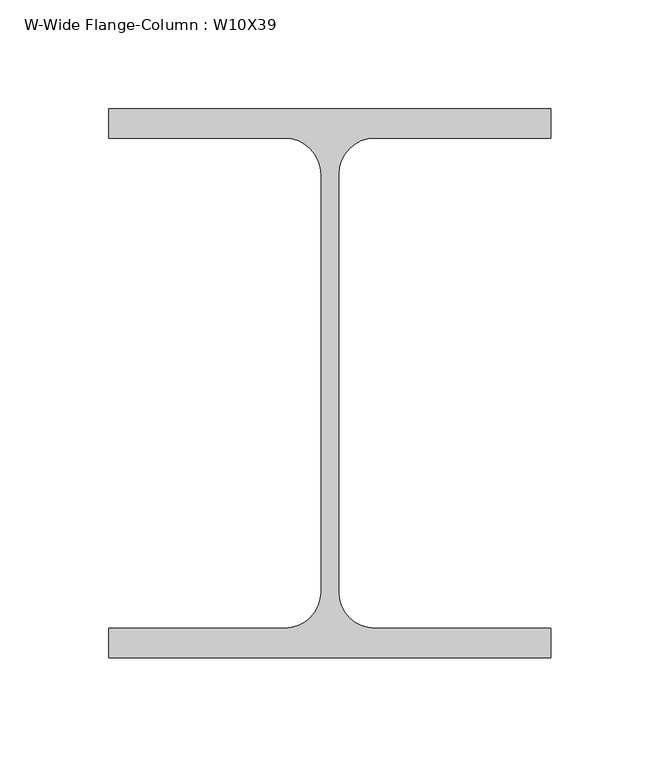
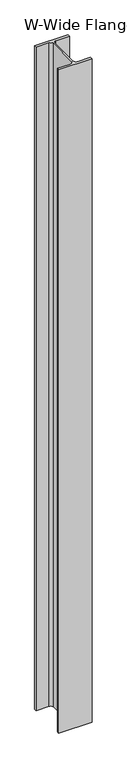
"""IFC4 building model written with IfcOpenShell, lengths in millimetres: column geometry, W-Wide Flange-Column : W10X39."""

from ifc_helpers import new_model, si_unit, point, frame, frame_2d, origin, place, context, project, spatial, polyline, circle_curve, trimmed, segment, composite_curve, outline, extrude, source, transform, mapped, element, save


def w_wide_flange_column_w10x39_5a593fdc(model_context):
    return source(origin(), model_context, "Body", "SweptSolid", [
        extrude(outline(composite_curve([segment(polyline([(101.473, 125.984), (101.473, 112.522), (20.701, 112.522)]), True, "CONTINUOUS"), segment(trimmed(circle_curve(frame_2d((20.701, 95.8215)), 16.7005), [point((20.701, 112.522))], [point((4.0005, 95.8215))], True, "CARTESIAN"), True, "CONTINUOUS"), segment(polyline([(4.0005, 95.8215), (4.0005, -95.8215)]), True, "CONTINUOUS"), segment(trimmed(circle_curve(frame_2d((20.701, -95.8215)), 16.7005), [point((4.0005, -95.8215))], [point((20.701, -112.522))], True, "CARTESIAN"), True, "CONTINUOUS"), segment(polyline([(20.701, -112.522), (101.473, -112.522), (101.473, -125.984), (-101.473, -125.984), (-101.473, -112.522), (-20.701, -112.522)]), True, "CONTINUOUS"), segment(trimmed(circle_curve(frame_2d((-20.701, -95.8215)), 16.7005), [point((-20.701, -112.522))], [point((-4.0005, -95.8215))], True, "CARTESIAN"), True, "CONTINUOUS"), segment(polyline([(-4.0005, -95.8215), (-4.0005, 95.8215)]), True, "CONTINUOUS"), segment(trimmed(circle_curve(frame_2d((-20.701, 95.8215)), 16.7005), [point((-4.0005, 95.8215))], [point((-20.701, 112.522))], True, "CARTESIAN"), True, "CONTINUOUS"), segment(polyline([(-20.701, 112.522), (-101.473, 112.522), (-101.473, 125.984), (101.473, 125.984)]), True, "CONTINUOUS")], self_intersect=False)), frame((0.0, 0.0, 23317.2), z_axis=(0.0, 0.0, 1.0), x_axis=(1.0, 0.0, 0.0)), (0.0, 0.0, 1.0), 4267.2),
    ])


if __name__ == "__main__":
    model = new_model("IFC4")
    model_context = context("Model", 3, world=origin())
    ifc_project = project(units=[si_unit("LENGTHUNIT", "METRE", prefix="MILLI")], contexts=[model_context])
    site = spatial("IfcSite", under=ifc_project)
    building = spatial("IfcBuilding", under=site)
    placement = place(None, origin())
    w_wide_flange_column_w10x39_shape = w_wide_flange_column_w10x39_5a593fdc(model_context)
    element("IfcColumn", 1, ObjectType="W-Wide Flange-Column : W10X39", at=placement, inside=building, context=model_context, shape_type="MappedRepresentation", body=[
        mapped(w_wide_flange_column_w10x39_shape, transform((0.0, 0.0, 0.0), x_axis=(1.0, 0.0, 0.0), y_axis=(0.0, 1.0, 0.0), z_axis=(0.0, 0.0, 1.0))),
    ])
    save(model, "model.ifc")

# Revit data of these elements
# Type "W-Wide Flange-Column : W10X39"
#   Assembly Code = "B10"
#   W = 39
#   bf = 0' - 7.99"
#   d = 0' - 9.92"
#   k = 0' - 1 3/16"
#   kr = 0' - 0.6575"
#   tf = 0' - 0.53"
#   tw = 0' - 0.315"
#   A = 0.0798611 SF
#   Structural Material [instance default] = Steel ASTM A992
# Element 1 (IfcColumn, "W-Wide Flange-Column : W10X39")
#   Materials on its faces: "Steel ASTM A992"
# Materials
#   "Steel ASTM A992": class "Metal", colour RGB 199 199 199, transparency 0, Description = "Structural steel 50ksi", Cost = 0
